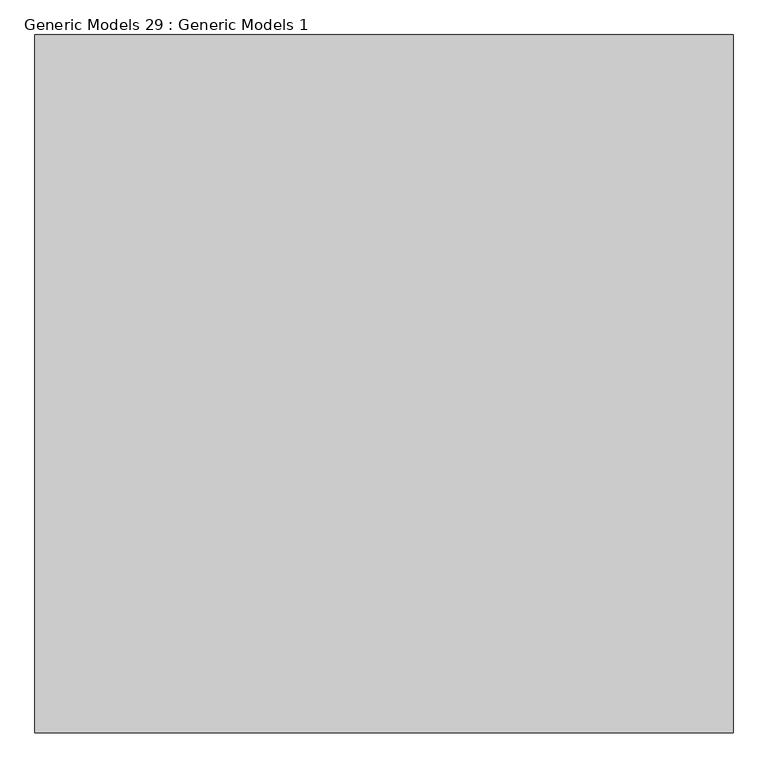
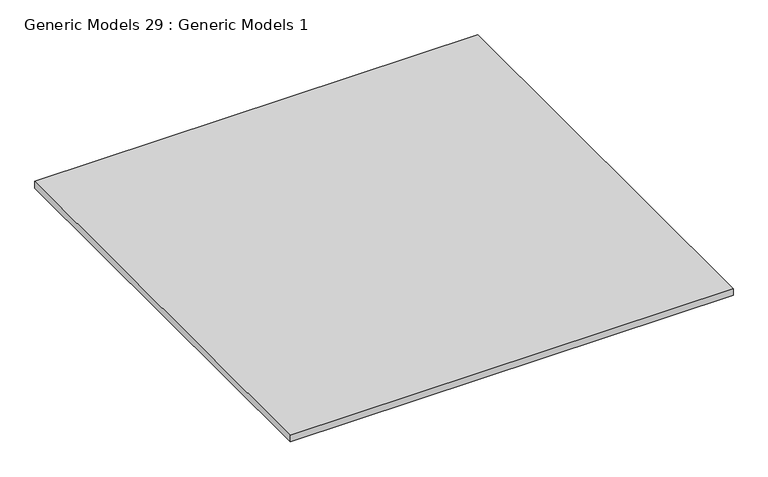
"""IFC4 building model written with IfcOpenShell, lengths in millimetres: proxy geometry, Generic Models 29 : Generic Models 1."""

from ifc_helpers import new_model, si_unit, frame, origin, place, context, project, spatial, polyline, outline, extrude, source, transform, mapped, element, save


def generic_models_29_generic_models_1_59087225(model_context):
    return source(origin(), model_context, "Body", "SweptSolid", [
        extrude(outline(polyline([(50347.5625, 1219.2), (50347.5625, 0.0), (49128.3625, 0.0), (49128.3625, 1219.2), (50347.5625, 1219.2)])), frame((0.0, 0.0, 5647.53125), z_axis=(0.0, 0.0, 1.0), x_axis=(1.0, 0.0, 0.0)), (0.0, 0.0, 1.0), 19.05),
    ])


if __name__ == "__main__":
    model = new_model("IFC4")
    model_context = context("Model", 3, world=origin())
    ifc_project = project(units=[si_unit("LENGTHUNIT", "METRE", prefix="MILLI")], contexts=[model_context])
    site = spatial("IfcSite", under=ifc_project)
    building = spatial("IfcBuilding", under=site)
    placement = place(None, origin())
    generic_models_29_generic_models_1_shape = generic_models_29_generic_models_1_59087225(model_context)
    element("IfcBuildingElementProxy", 1, Name="Generic Models 29 : Generic Models 1", ObjectType="Generic Models 29 : Generic Models 1", at=placement, inside=building, context=model_context, shape_type="MappedRepresentation", body=[
        mapped(generic_models_29_generic_models_1_shape, transform((0.0, 0.0, 0.0), x_axis=(1.0, 0.0, 0.0), y_axis=(0.0, 1.0, 0.0), z_axis=(0.0, 0.0, 1.0))),
    ])
    save(model, "model.ifc")

# Revit data of these elements
# Element 1 (IfcBuildingElementProxy, "Generic Models 29 : Generic Models 1")
#   Materials on its faces: "SUBSTRATE AS SCHEDULED"
# Materials
#   "SUBSTRATE AS SCHEDULED": class "Unassigned", colour RGB 196 177 123, transparency 0, Cost = 0
